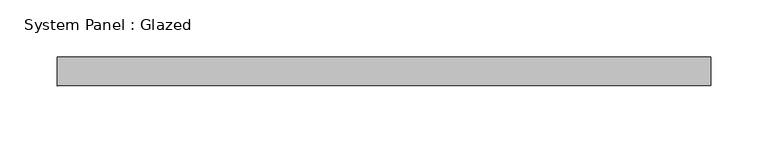
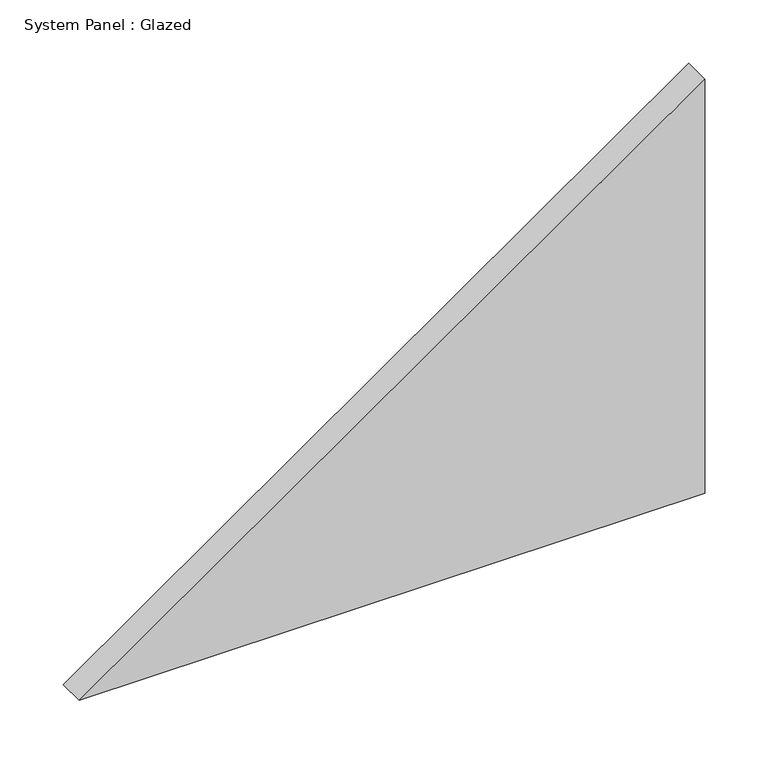
"""IFC4 building model written with IfcOpenShell, lengths in millimetres: plate geometry, System Panel : Glazed."""

from ifc_helpers import new_model, si_unit, frame, origin, place, context, project, spatial, polyline, outline, extrude, source, transform, mapped, element, save


def system_panel_glazed_9091093d(model_context):
    return source(origin(), model_context, "Body", "SweptSolid", [
        extrude(outline(polyline([(0.0, -285.117578), (0.0, 285.117578), (399.2829548, 285.117578), (0.0, -285.117578)])), frame((0.0, -49.5, 0.0), z_axis=(0.0, 1.0, 0.0), x_axis=(0.0, 0.0, 1.0)), (0.0, 0.0, 1.0), 25.0),
    ])


if __name__ == "__main__":
    model = new_model("IFC4")
    model_context = context("Model", 3, world=origin())
    ifc_project = project(units=[si_unit("LENGTHUNIT", "METRE", prefix="MILLI")], contexts=[model_context])
    site = spatial("IfcSite", under=ifc_project)
    building = spatial("IfcBuilding", under=site)
    placement = place(None, origin())
    system_panel_glazed_shape = system_panel_glazed_9091093d(model_context)
    element("IfcPlate", 1, ObjectType="System Panel : Glazed", at=placement, inside=building, context=model_context, shape_type="MappedRepresentation", body=[
        mapped(system_panel_glazed_shape, transform((0.0, 0.0, 0.0), x_axis=(1.0, 0.0, 0.0), y_axis=(0.0, 1.0, 0.0), z_axis=(0.0, 0.0, 1.0))),
    ])
    save(model, "model.ifc")

# Revit data of these elements
# Type "System Panel : Glazed"
#   Construction Type Id = "GSP4R"
#   Analytic Construction = "1/8 in Pilkington single glazing"
#   Visual Light Transmittance = 0.9
#   Solar Heat Gain Coefficient = 0.86
#   Heat Transfer Coefficient (U) = 6.7069 W/(m²·K)
#   Define Thermal Properties by = 1
# Element 1 (IfcPlate, "System Panel : Glazed")
#   Materials on its faces: "Glass"
# Materials
#   "Glass": class "Glass", colour RGB 0 128 192, transparency 0.9, Description = "Soda Lime Glass", Cost = 0
